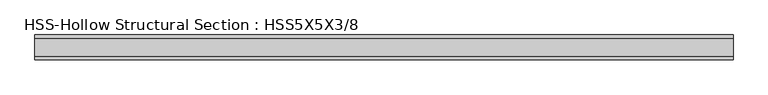
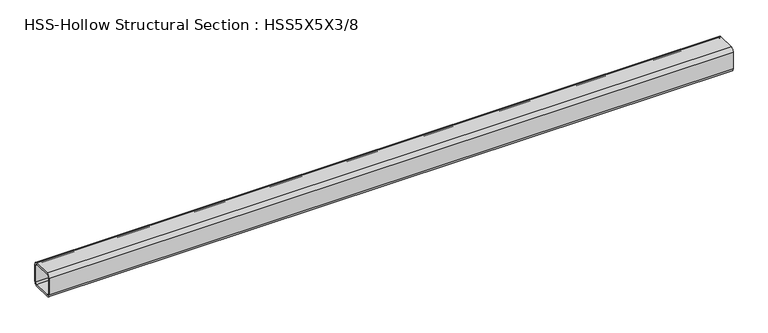
"""IFC4 building model written with IfcOpenShell, lengths in millimetres: member geometry, HSS-Hollow Structural Section : HSS5X5X3/8."""

import ifcopenshell
import ifcopenshell.guid

model = None  # the IFC model being written
_history = None  # IfcOwnerHistory: only IFC2X3 demands one
_inside = {}  # id of a spatial element -> (the spatial element, [elements in it])
_under = {}  # id of a project, library or spatial element -> (it, [spatial elements below it])
_declared = {}  # id of a project -> (the project, [libraries it declares])
_typed = {}  # id of a type object -> (the type object, [elements of that type])
_made_of = {}  # id of a material, layer set ... -> (it, [elements and type objects made of it])


def new_model(schema):
    """Start an empty IFC model of exactly this schema.

    Asked for "IFC4X3", IfcOpenShell would pick the latest addendum, in which some entities
    have other attributes; the version numbers below select the first issue.
    IFC2X3 requires an IfcOwnerHistory on every rooted entity: one is made here for all.
    """
    global model, _history
    if schema == "IFC4X3":
        model = ifcopenshell.file(schema_version=(4, 3, 0, 0))
    else:
        model = ifcopenshell.file(schema=schema)
    _inside.clear()
    _under.clear()
    _declared.clear()
    _typed.clear()
    _made_of.clear()
    _history = None
    if model.schema == "IFC2X3":
        org = make("IfcOrganization", Name="unknown")
        user = make(
            "IfcPersonAndOrganization",
            ThePerson=make("IfcPerson", FamilyName="unknown"),
            TheOrganization=org,
        )
        app = make(
            "IfcApplication",
            ApplicationDeveloper=org,
            Version="unknown",
            ApplicationFullName="unknown",
            ApplicationIdentifier="unknown",
        )
        _history = make(
            "IfcOwnerHistory",
            OwningUser=user,
            OwningApplication=app,
            ChangeAction="ADDED",
            CreationDate=0,
        )
    return model


def make(cls, **values):
    """One entity of the class cls with the attributes given. An attribute that is None is left unset."""
    return model.create_entity(
        cls, **{name: value for name, value in values.items() if value is not None}
    )


def rooted(cls, **values):
    """An entity with a GlobalId (a new one), such as an element, a storey or a relation."""
    return make(cls, GlobalId=ifcopenshell.guid.new(), OwnerHistory=_history, **values)


def si_unit(unit_type, name, prefix=None):
    """IfcSIUnit, for example si_unit("LENGTHUNIT", "METRE", prefix="MILLI")."""
    return make("IfcSIUnit", UnitType=unit_type, Prefix=prefix, Name=name)


def assignment(units):
    """IfcUnitAssignment: the units of a project."""
    return None if units is None else make("IfcUnitAssignment", Units=units)


def point(xyz):
    """IfcCartesianPoint."""
    return None if xyz is None else make("IfcCartesianPoint", Coordinates=xyz)


def direction(xyz):
    """IfcDirection."""
    return None if xyz is None else make("IfcDirection", DirectionRatios=xyz)


def frame(location, z_axis=None, x_axis=None):
    """IfcAxis2Placement3D, a coordinate frame: its origin and axes. An axis left out is left unset."""
    return make(
        "IfcAxis2Placement3D",
        Location=point(location),
        Axis=direction(z_axis),
        RefDirection=direction(x_axis),
    )


def frame_2d(location, x_axis=None):
    """IfcAxis2Placement2D, a coordinate frame in the plane: its origin and x axis."""
    return make(
        "IfcAxis2Placement2D", Location=point(location), RefDirection=direction(x_axis)
    )


def origin():
    """The frame at (0, 0, 0) with its axes left unset."""
    return frame((0.0, 0.0, 0.0))


def place(relative_to, where):
    """IfcLocalPlacement: puts the frame where relative to a parent placement (None: the world)."""
    return make(
        "IfcLocalPlacement", PlacementRelTo=relative_to, RelativePlacement=where
    )


def context(
    kind, dimensions, precision=None, world=None, true_north=None, identifier=None
):
    """IfcGeometricRepresentationContext, for example the 3D "Model" context."""
    return make(
        "IfcGeometricRepresentationContext",
        ContextIdentifier=identifier,
        ContextType=kind,
        CoordinateSpaceDimension=dimensions,
        Precision=precision,
        WorldCoordinateSystem=world,
        TrueNorth=true_north,
    )


def project(units=None, contexts=None):
    """IfcProject with its units and contexts."""
    return rooted(
        "IfcProject",
        Name="project",
        RepresentationContexts=contexts,
        UnitsInContext=assignment(units),
    )


def spatial(cls, under=None, at=None, **own):
    """A site, building, storey or space (cls), placed at a placement, below another one or the project."""
    s = rooted(cls, ObjectPlacement=at, **own)
    if under is not None:
        _under.setdefault(under.id(), (under, []))[1].append(s)
    return s


def polyline(points):
    """IfcPolyline through the points."""
    return make("IfcPolyline", Points=[point(p) for p in points])


def circle_curve(where, radius):
    """IfcCircle in the frame where."""
    return make("IfcCircle", Position=where, Radius=radius)


def trimmed(basis, trim1, trim2, sense, master):
    """IfcTrimmedCurve: the piece of a basis curve between two trims."""
    return make(
        "IfcTrimmedCurve",
        BasisCurve=basis,
        Trim1=trim1,
        Trim2=trim2,
        SenseAgreement=sense,
        MasterRepresentation=master,
    )


def segment(curve, same_sense, transition):
    """IfcCompositeCurveSegment."""
    return make(
        "IfcCompositeCurveSegment",
        Transition=transition,
        SameSense=same_sense,
        ParentCurve=curve,
    )


def composite_curve(segments, self_intersect=None):
    """IfcCompositeCurve: segments joined end to end."""
    return make("IfcCompositeCurve", Segments=segments, SelfIntersect=self_intersect)


def outline(outer, holes=None, kind="AREA"):
    """IfcArbitraryClosedProfileDef: a profile drawn as a closed curve; with holes, ...WithVoids."""
    if holes is None:
        return make("IfcArbitraryClosedProfileDef", ProfileType=kind, OuterCurve=outer)
    return make(
        "IfcArbitraryProfileDefWithVoids",
        ProfileType=kind,
        OuterCurve=outer,
        InnerCurves=holes,
    )


def extrude(swept, where, along, depth):
    """IfcExtrudedAreaSolid: the profile swept, set in the frame where, extruded along a direction by depth."""
    return make(
        "IfcExtrudedAreaSolid",
        SweptArea=swept,
        Position=where,
        ExtrudedDirection=direction(along),
        Depth=depth,
    )


def shape(context_of_items, identifier, shape_type, items):
    """IfcShapeRepresentation: the items that make up one representation, for example the "Body"."""
    return make(
        "IfcShapeRepresentation",
        ContextOfItems=context_of_items,
        RepresentationIdentifier=identifier,
        RepresentationType=shape_type,
        Items=items,
    )


def source(mapping_origin, context_of_items, identifier, shape_type, items):
    """IfcRepresentationMap: a shape defined once, which mapped items show again and again."""
    return make(
        "IfcRepresentationMap",
        MappingOrigin=mapping_origin,
        MappedRepresentation=shape(context_of_items, identifier, shape_type, items),
    )


def transform(
    local_origin,
    x_axis=None,
    y_axis=None,
    z_axis=None,
    scale=None,
    scale2=None,
    scale3=None,
    uniform=True,
):
    """IfcCartesianTransformationOperator3D, or its non-uniform kind. x_axis, y_axis, z_axis: its Axis1, 2, 3."""
    if uniform:
        return make(
            "IfcCartesianTransformationOperator3D",
            Axis1=direction(x_axis),
            Axis2=direction(y_axis),
            LocalOrigin=point(local_origin),
            Scale=scale,
            Axis3=direction(z_axis),
        )
    return make(
        "IfcCartesianTransformationOperator3DnonUniform",
        Axis1=direction(x_axis),
        Axis2=direction(y_axis),
        LocalOrigin=point(local_origin),
        Scale=scale,
        Axis3=direction(z_axis),
        Scale2=scale2,
        Scale3=scale3,
    )


def mapped(mapping_source, mapping_target):
    """IfcMappedItem: shows the shape of a source again, moved by a transform."""
    return make(
        "IfcMappedItem", MappingSource=mapping_source, MappingTarget=mapping_target
    )


def made_of(thing, what):
    """Note that an element or type object is made of a material, layer set ...; save() writes the relation."""
    if what is not None:
        _made_of.setdefault(what.id(), (what, []))[1].append(thing)
    return thing


def element(
    cls,
    number,
    at=None,
    inside=None,
    cuts=None,
    type_object=None,
    material=None,
    context=None,
    identifier="Body",
    shape_type=None,
    held_by="IfcProductDefinitionShape",
    body=None,
    shapes=None,
    **own,
):
    """One element of the class cls, such as IfcWall. Its Tag is "e" and its number.

    at: its placement. inside: the storey or other place that contains it. cuts: it is an
    opening in that element (IfcRelVoidsElement). A single representation is given by context,
    identifier, shape_type and body (its items); several are given by shapes. held_by: the class
    of the entity that holds the representations. save() writes the other relations.
    """
    e = rooted(cls, Tag="e%d" % number, ObjectPlacement=at, **own)
    if body is not None:
        shapes = [shape(context, identifier, shape_type, body)]
    if shapes is not None:
        e.Representation = make(held_by, Representations=shapes)
    if inside is not None:
        _inside.setdefault(inside.id(), (inside, []))[1].append(e)
    if cuts is not None:
        rooted(
            "IfcRelVoidsElement", RelatingBuildingElement=cuts, RelatedOpeningElement=e
        )
    if type_object is not None:
        _typed.setdefault(type_object.id(), (type_object, []))[1].append(e)
    return made_of(e, material)


def aggregate(whole, parts):
    """IfcRelAggregates: a whole, such as a stair, and the parts it consists of."""
    return rooted("IfcRelAggregates", RelatingObject=whole, RelatedObjects=parts)


def save(model, path):
    """Write the relations noted so far, then the file.

    IfcRelAggregates (storeys below a building ...), IfcRelContainedInSpatialStructure (elements
    in a storey), IfcRelDefinesByType, IfcRelAssociatesMaterial and IfcRelDeclares: one each for
    every whole, place, type object, material and project.
    """
    for whole, parts in _under.values():
        aggregate(whole, parts)
    for where, things in _inside.values():
        rooted(
            "IfcRelContainedInSpatialStructure",
            RelatedElements=things,
            RelatingStructure=where,
        )
    for kind, things in _typed.values():
        rooted("IfcRelDefinesByType", RelatedObjects=things, RelatingType=kind)
    for what, things in _made_of.values():
        rooted("IfcRelAssociatesMaterial", RelatedObjects=things, RelatingMaterial=what)
    for by, libraries in _declared.values():
        rooted("IfcRelDeclares", RelatingContext=by, RelatedDefinitions=libraries)
    model.write(path)


def hss_hollow_structural_section_hss5x5x3_8_2df68ff6(model_context):
    return source(origin(), model_context, "Body", "SweptSolid", [
        extrude(outline(composite_curve([segment(polyline([(63.5, 45.7708), (63.5, -45.7708)]), True, "CONTINUOUS"), segment(trimmed(circle_curve(frame_2d((45.7708, -45.7708)), 17.7292), [point((63.5, -45.7708))], [point((45.7708, -63.5))], False, "CARTESIAN"), True, "CONTINUOUS"), segment(polyline([(45.7708, -63.5), (-45.7708, -63.5)]), True, "CONTINUOUS"), segment(trimmed(circle_curve(frame_2d((-45.7708, -45.7708)), 17.7292), [point((-45.7708, -63.5))], [point((-63.5, -45.7708))], False, "CARTESIAN"), True, "CONTINUOUS"), segment(polyline([(-63.5, -45.7708), (-63.5, 45.7708)]), True, "CONTINUOUS"), segment(trimmed(circle_curve(frame_2d((-45.7708, 45.7708)), 17.7292), [point((-63.5, 45.7708))], [point((-45.7708, 63.5))], False, "CARTESIAN"), True, "CONTINUOUS"), segment(polyline([(-45.7708, 63.5), (45.7708, 63.5)]), True, "CONTINUOUS"), segment(trimmed(circle_curve(frame_2d((45.7708, 45.7708)), 17.7292), [point((45.7708, 63.5))], [point((63.5, 45.7708))], False, "CARTESIAN"), True, "CONTINUOUS")], self_intersect=False), holes=[composite_curve([segment(trimmed(circle_curve(frame_2d((-45.7708, 45.7708)), 8.8646), [point((-45.7708, 54.6354))], [point((-54.6354, 45.7708))], True, "CARTESIAN"), True, "CONTINUOUS"), segment(polyline([(-54.6354, 45.7708), (-54.6354, -45.7708)]), True, "CONTINUOUS"), segment(trimmed(circle_curve(frame_2d((-45.7708, -45.7708)), 8.8646), [point((-54.6354, -45.7708))], [point((-45.7708, -54.6354))], True, "CARTESIAN"), True, "CONTINUOUS"), segment(polyline([(-45.7708, -54.6354), (45.7708, -54.6354)]), True, "CONTINUOUS"), segment(trimmed(circle_curve(frame_2d((45.7708, -45.7708)), 8.8646), [point((45.7708, -54.6354))], [point((54.6354, -45.7708))], True, "CARTESIAN"), True, "CONTINUOUS"), segment(polyline([(54.6354, -45.7708), (54.6354, 45.7708)]), True, "CONTINUOUS"), segment(trimmed(circle_curve(frame_2d((45.7708, 45.7708)), 8.8646), [point((54.6354, 45.7708))], [point((45.7708, 54.6354))], True, "CARTESIAN"), True, "CONTINUOUS"), segment(polyline([(45.7708, 54.6354), (-45.7708, 54.6354)]), True, "CONTINUOUS")], self_intersect=False)]), frame((-1778.3838811, 0.0, 0.0), z_axis=(1.0, 0.0, 0.0), x_axis=(0.0, 1.0, 0.0)), (0.0, 0.0, 1.0), 3556.7677621),
    ])


if __name__ == "__main__":
    model = new_model("IFC4")
    model_context = context("Model", 3, world=origin())
    ifc_project = project(units=[si_unit("LENGTHUNIT", "METRE", prefix="MILLI")], contexts=[model_context])
    site = spatial("IfcSite", under=ifc_project)
    building = spatial("IfcBuilding", under=site)
    placement = place(None, origin())
    hss_hollow_structural_section_hss5x5x3_8_shape = hss_hollow_structural_section_hss5x5x3_8_2df68ff6(model_context)
    element("IfcMember", 1, ObjectType="HSS-Hollow Structural Section : HSS5X5X3/8", at=placement, inside=building, context=model_context, shape_type="MappedRepresentation", body=[
        mapped(hss_hollow_structural_section_hss5x5x3_8_shape, transform((0.0, 0.0, 0.0), x_axis=(1.0, 0.0, 0.0), y_axis=(0.0, 1.0, 0.0), z_axis=(0.0, 0.0, 1.0))),
    ])
    save(model, "model.ifc")

# Revit data of these elements
# Type "HSS-Hollow Structural Section : HSS5X5X3/8"
#   Assembly Code = "B10"
#   Shape = "Square"
#   W = 22.3
#   Ht = 0' - 5"
#   Length [instance default] = 5' - 0"
#   b = 0' - 5"
#   kr = 0' - 0.698"
#   t = 0' - 0.349"
#   A = 0.0429167 SF
#   Structural Material [instance default] = Steel ASTM A500, Grade B, Rectangular and Square
# Element 1 (IfcMember, "HSS-Hollow Structural Section : HSS5X5X3/8")
#   Materials on its faces: "Steel ASTM A500, Grade B, Rectangular and Square"
# Materials
#   "Steel ASTM A500, Grade B, Rectangular and Square": class "Metal", colour RGB 199 199 199, transparency 0, Description = "Carbon steel", Cost = 0
